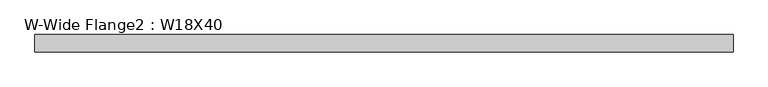
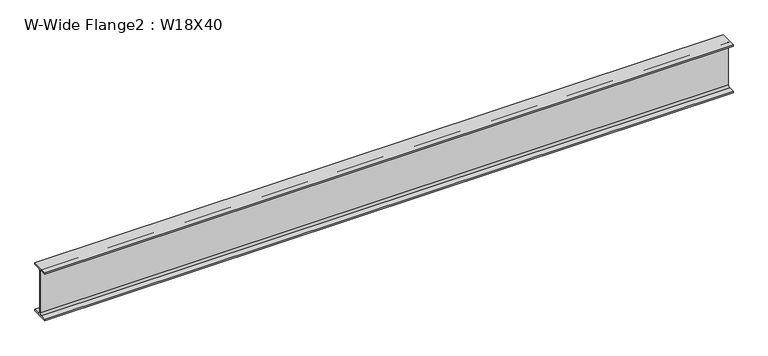
"""IFC4 building model written with IfcOpenShell, lengths in millimetres: beam geometry, W-Wide Flange2 : W18X40."""

from ifc_helpers import new_model, si_unit, point, frame, frame_2d, origin, place, context, project, spatial, polyline, circle_curve, trimmed, segment, composite_curve, outline, extrude, source, transform, mapped, element, save


def w_wide_flange2_w18x40_9a74fa6d(model_context):
    return source(origin(), model_context, "Body", "SweptSolid", [
        extrude(outline(composite_curve([segment(polyline([(76.454, -213.995), (76.454, -227.33), (-76.454, -227.33), (-76.454, -213.995), (-20.828, -213.995)]), True, "CONTINUOUS"), segment(trimmed(circle_curve(frame_2d((-20.828, -197.1675)), 16.8275), [point((-20.828, -213.995))], [point((-4.0005, -197.1675))], True, "CARTESIAN"), True, "CONTINUOUS"), segment(polyline([(-4.0005, -197.1675), (-4.0005, 197.1675)]), True, "CONTINUOUS"), segment(trimmed(circle_curve(frame_2d((-20.828, 197.1675)), 16.8275), [point((-4.0005, 197.1675))], [point((-20.828, 213.995))], True, "CARTESIAN"), True, "CONTINUOUS"), segment(polyline([(-20.828, 213.995), (-76.454, 213.995), (-76.454, 227.33), (76.454, 227.33), (76.454, 213.995), (20.828, 213.995)]), True, "CONTINUOUS"), segment(trimmed(circle_curve(frame_2d((20.828, 197.1675)), 16.8275), [point((20.828, 213.995))], [point((4.0005, 197.1675))], True, "CARTESIAN"), True, "CONTINUOUS"), segment(polyline([(4.0005, 197.1675), (4.0005, -197.1675)]), True, "CONTINUOUS"), segment(trimmed(circle_curve(frame_2d((20.828, -197.1675)), 16.8275), [point((4.0005, -197.1675))], [point((20.828, -213.995))], True, "CARTESIAN"), True, "CONTINUOUS"), segment(polyline([(20.828, -213.995), (76.454, -213.995)]), True, "CONTINUOUS")], self_intersect=False)), frame((-3084.5125, 0.0, 0.0), z_axis=(1.0, 0.0, 0.0), x_axis=(0.0, 1.0, 0.0)), (0.0, 0.0, 1.0), 6169.025),
    ])


if __name__ == "__main__":
    model = new_model("IFC4")
    model_context = context("Model", 3, world=origin())
    ifc_project = project(units=[si_unit("LENGTHUNIT", "METRE", prefix="MILLI")], contexts=[model_context])
    site = spatial("IfcSite", under=ifc_project)
    building = spatial("IfcBuilding", under=site)
    placement = place(None, origin())
    w_wide_flange2_w18x40_shape = w_wide_flange2_w18x40_9a74fa6d(model_context)
    element("IfcBeam", 1, ObjectType="W-Wide Flange2 : W18X40", at=placement, inside=building, context=model_context, shape_type="MappedRepresentation", body=[
        mapped(w_wide_flange2_w18x40_shape, transform((0.0, 0.0, 0.0), x_axis=(1.0, 0.0, 0.0), y_axis=(0.0, 1.0, 0.0), z_axis=(0.0, 0.0, 1.0))),
    ])
    save(model, "model.ifc")

# Revit data of these elements
# Type "W-Wide Flange2 : W18X40"
#   Assembly Code = "B10"
#   W = 40
#   Length [instance default] = 5' - 0"
#   bf = 0' - 6.02"
#   d = 1' - 5.9"
#   k = 0' - 1 3/16"
#   k2 = 0' - 0.6625"
#   tf = 0' - 0.525"
#   tw = 0' - 0.315"
#   A = 0.0819444 SF
#   Structural Material [instance default] = Steel ASTM A992
# Element 1 (IfcBeam, "W-Wide Flange2 : W18X40")
#   Materials on its faces: "Steel ASTM A992"
# Materials
#   "Steel ASTM A992": class "Metal", colour RGB 199 199 199, transparency 0, Description = "Structural steel 50ksi", Cost = 0
